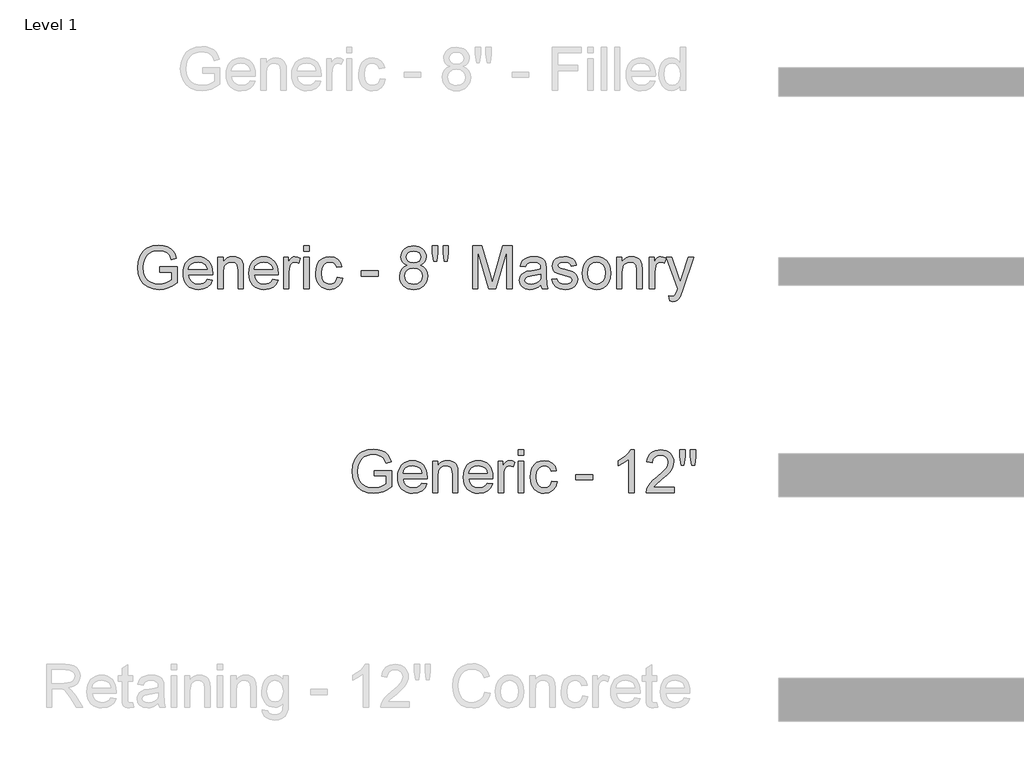
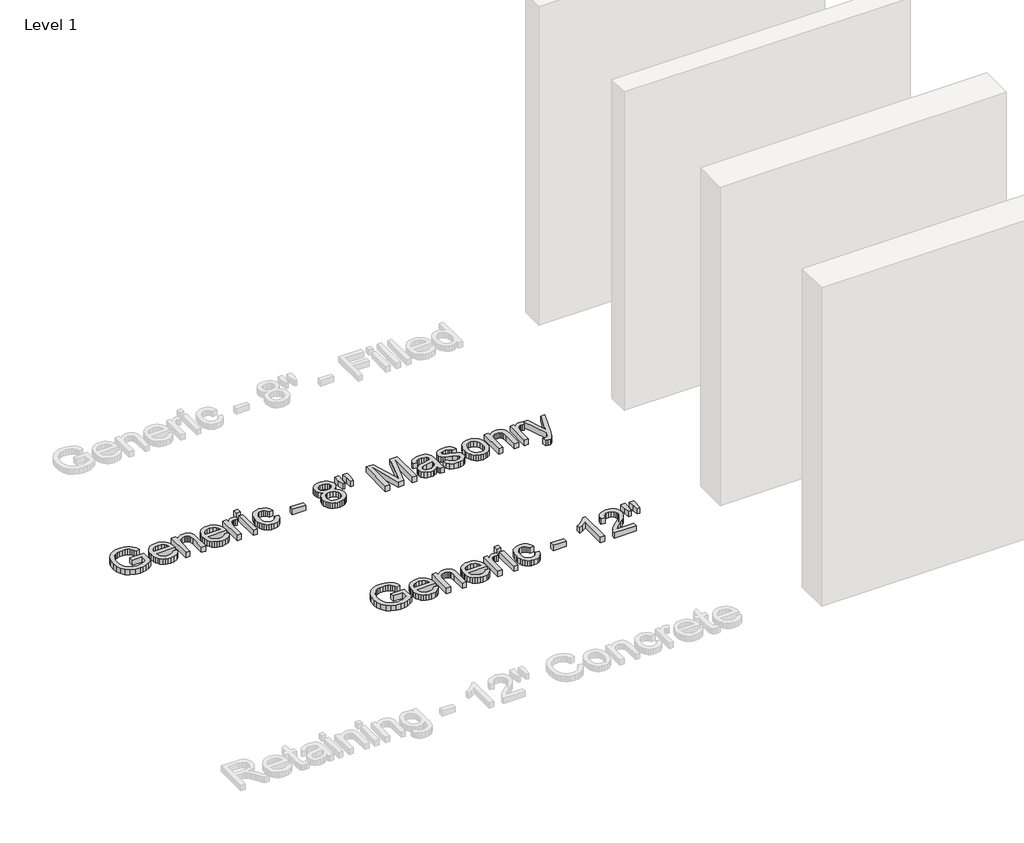
# One storey, part 22 of 42: 2 proxies.
"""IFC4 building model written with IfcOpenShell, lengths in millimetres."""

from ifc_helpers import new_model, si_unit, origin, origin_with_axes, place, context, project, spatial, polyline, outline, extrude, element, save

model = new_model("IFC4")

# Units and contexts
model_context = context("Model", 3, world=origin())
ifc_project = project(units=[si_unit("LENGTHUNIT", "METRE", prefix="MILLI")], contexts=[model_context])

# Site, building, storey
site = spatial("IfcSite", under=ifc_project)
building = spatial("IfcBuilding", under=site)
storey = spatial("IfcBuildingStorey", under=building, Name="Level 1", Elevation=0.0)

# Proxies
placement = place(None, origin())
element("IfcBuildingElementProxy", 1, Name="8\" Arial", ObjectType="8\" Arial", at=placement, inside=storey, context=model_context, shape_type="SweptSolid", body=[
    extrude(outline(polyline([(-16920.0716605, 9639.2549176), (-16920.0716605, 9677.3258044), (-16796.3412786, 9677.3258044), (-16796.3412786, 9563.4849301), (-16826.4094716, 9542.5719674), (-16857.4257189, 9527.5704021), (-16889.3156634, 9518.5360023), (-16922.0049477, 9515.5245356), (-16964.7138649, 9520.3112804), (-17003.3145467, 9534.6715148), (-17035.3810895, 9558.1033277), (-17058.4875896, 9590.1048079), (-17072.4574487, 9628.4917128), (-17077.1140684, 9671.0797995), (-17072.476038, 9713.9746097), (-17058.5619468, 9753.8765425), (-17035.9480632, 9787.3465774), (-17021.5947998, 9800.3800005), (-17005.2106553, 9810.945694), (-16967.7718048, 9824.943437), (-16925.053593, 9829.6093514), (-16893.6934436, 9826.9046082), (-16865.4934752, 9818.7903787), (-16841.7456442, 9805.8522258), (-16823.741907, 9788.6757124), (-16810.4226734, 9766.4336147), (-16800.7283534, 9738.2987089), (-16835.8249521, 9728.4092012), (-16843.6603421, 9748.4763508), (-16853.1873585, 9763.6173358), (-16865.790904, 9775.0311661), (-16882.8558816, 9783.9168516), (-16903.2018706, 9789.6330614), (-16925.6484506, 9791.5384646), (-16951.9244264, 9789.484347), (-16974.3895956, 9783.321994), (-16992.9603065, 9773.8228616), (-17007.5529071, 9761.7584058), (-17027.1460295, 9732.4244901), (-17036.0688936, 9703.685432), (-17039.0431816, 9672.6413007), (-17035.4647414, 9636.2341563), (-17024.7294205, 9606.2774991), (-17007.1625318, 9582.985106), (-16983.0893881, 9566.5707539), (-16954.9173037, 9556.8392553), (-16925.053593, 9553.5954224), (-16898.6846707, 9556.0399154), (-16872.9663739, 9563.3733943), (-16850.6313297, 9573.4766789), (-16834.4121653, 9584.2305891), (-16834.4121653, 9639.2549176), (-16920.0716605, 9639.2549176)])), origin_with_axes(), (0.0, 0.0, 1.0), 50.8),
    extrude(outline(polyline([(-16582.6386837, 9586.9074483), (-16545.311369, 9582.1485875), (-16558.7607277, 9554.0229763), (-16580.2220747, 9532.9984778), (-16609.2120883, 9519.8930212), (-16645.2474467, 9515.5245356), (-16668.8697999, 9517.4090259), (-16689.917535, 9523.0624969), (-16708.3906521, 9532.4849484), (-16724.2891511, 9545.6763805), (-16737.0739423, 9562.2696546), (-16746.205936, 9581.8976319), (-16751.6851322, 9604.5603125), (-16753.5115309, 9630.2576963), (-16751.6665429, 9656.8264536), (-16746.1315788, 9680.2443245), (-16736.9066386, 9700.511309), (-16723.9917223, 9717.6274071), (-16708.1350492, 9731.2254802), (-16690.0848387, 9740.9383896), (-16669.8410909, 9746.7661352), (-16647.4038055, 9748.708717), (-16625.6891793, 9746.7707825), (-16606.0519073, 9740.9569789), (-16588.4919896, 9731.2673061), (-16573.0094262, 9717.7017643), (-16560.3710258, 9700.6228448), (-16551.3435969, 9680.3930389), (-16545.9271396, 9657.0123466), (-16544.1216538, 9630.4807679), (-16544.3447254, 9620.2194742), (-16715.4406442, 9620.2194742), (-16708.8507373, 9591.722077), (-16693.5424486, 9570.7719358), (-16671.4490653, 9557.8895507), (-16644.5038747, 9553.5954224), (-16624.2415375, 9555.5844775), (-16607.17656, 9561.5516429), (-16593.308942, 9571.8687045), (-16582.6386837, 9586.9074483)]), holes=[polyline([(-16715.4406442, 9658.290361), (-16582.1925405, 9658.290361), (-16587.3417767, 9678.4039838), (-16597.4357667, 9692.7921021), (-16619.6313911, 9706.1763982), (-16647.5525199, 9710.6378303), (-16673.2150488, 9707.0779793), (-16694.434735, 9696.3984263), (-16709.1853447, 9679.751708), (-16715.4406442, 9658.290361)])]), origin_with_axes(), (0.0, 0.0, 1.0), 50.8),
    extrude(outline(polyline([(-16506.050767, 9520.2833965), (-16506.050767, 9743.9498562), (-16467.9798803, 9743.9498562), (-16467.9798803, 9712.7198319), (-16454.7535932, 9728.4649691), (-16438.8690362, 9739.7114957), (-16420.3262093, 9746.4594117), (-16399.1251124, 9748.708717), (-16380.3592139, 9746.8962603), (-16363.1734059, 9741.45889), (-16348.8410554, 9733.0751156), (-16338.6355296, 9722.4234466), (-16327.2216993, 9694.4279605), (-16325.2140549, 9657.6211462), (-16325.2140549, 9520.2833965), (-16363.2849417, 9520.2833965), (-16363.2849417, 9652.4904993), (-16367.6720165, 9686.1743112), (-16373.741423, 9696.2032387), (-16383.1754929, 9703.9828608), (-16395.2678326, 9708.9740879), (-16409.3120489, 9710.6378303), (-16431.6099145, 9706.9013809), (-16450.6174739, 9695.6920329), (-16458.2135267, 9686.5414499), (-16463.6392787, 9674.0354982), (-16467.9798803, 9638.9574888), (-16467.9798803, 9520.2833965), (-16506.050767, 9520.2833965)])), origin_with_axes(), (0.0, 0.0, 1.0), 50.8),
    extrude(outline(polyline([(-16116.2703209, 9586.9074483), (-16078.9430062, 9582.1485875), (-16092.3923649, 9554.0229763), (-16113.8537119, 9532.9984778), (-16142.8437255, 9519.8930212), (-16178.8790839, 9515.5245356), (-16202.5014371, 9517.4090259), (-16223.5491723, 9523.0624969), (-16242.0222893, 9532.4849484), (-16257.9207883, 9545.6763805), (-16270.7055795, 9562.2696546), (-16279.8375732, 9581.8976319), (-16285.3167694, 9604.5603125), (-16287.1431682, 9630.2576963), (-16285.2981801, 9656.8264536), (-16279.763216, 9680.2443245), (-16270.5382758, 9700.511309), (-16257.6233595, 9717.6274071), (-16241.7666864, 9731.2254802), (-16223.716476, 9740.9383896), (-16203.4727281, 9746.7661352), (-16181.0354428, 9748.708717), (-16159.3208165, 9746.7707825), (-16139.6835445, 9740.9569789), (-16122.1236268, 9731.2673061), (-16106.6410635, 9717.7017643), (-16094.002663, 9700.6228448), (-16084.9752341, 9680.3930389), (-16079.5587768, 9657.0123466), (-16077.753291, 9630.4807679), (-16077.9763626, 9620.2194742), (-16249.0722814, 9620.2194742), (-16242.4823745, 9591.722077), (-16227.1740858, 9570.7719358), (-16205.0807025, 9557.8895507), (-16178.1355119, 9553.5954224), (-16157.8731747, 9555.5844775), (-16140.8081972, 9561.5516429), (-16126.9405792, 9571.8687045), (-16116.2703209, 9586.9074483)]), holes=[polyline([(-16249.0722814, 9658.290361), (-16115.8241777, 9658.290361), (-16120.9734139, 9678.4039838), (-16131.0674039, 9692.7921021), (-16153.2630283, 9706.1763982), (-16181.1841572, 9710.6378303), (-16206.846686, 9707.0779793), (-16228.0663722, 9696.3984263), (-16242.8169819, 9679.751708), (-16249.0722814, 9658.290361)])]), origin_with_axes(), (0.0, 0.0, 1.0), 50.8),
    extrude(outline(polyline([(-16039.6824042, 9520.2833965), (-16039.6824042, 9743.9498562), (-16006.3703783, 9743.9498562), (-16006.3703783, 9710.8609019), (-15994.0642616, 9730.0450597), (-15982.7247885, 9741.3473542), (-15971.3481368, 9746.8683763), (-15958.9304843, 9748.708717), (-15939.9693981, 9745.7716076), (-15920.7108831, 9736.9602793), (-15933.4259644, 9702.8303242), (-15946.8102605, 9708.6859538), (-15960.1945567, 9710.6378303), (-15971.5619137, 9708.760311), (-15981.7209663, 9703.127753), (-15989.9281423, 9694.1677103), (-15995.4398698, 9682.3077368), (-16000.0686056, 9661.0415774), (-16001.6115175, 9637.8421308), (-16001.6115175, 9520.2833965), (-16039.6824042, 9520.2833965)])), origin_with_axes(), (0.0, 0.0, 1.0), 50.8),
    extrude(outline(polyline([(-15896.9165789, 9786.7796038), (-15896.9165789, 9824.8504905), (-15858.8456921, 9824.8504905), (-15858.8456921, 9786.7796038), (-15896.9165789, 9786.7796038)])), origin_with_axes(), (0.0, 0.0, 1.0), 50.8),
    extrude(outline(polyline([(-15896.9165789, 9520.2833965), (-15896.9165789, 9743.9498562), (-15858.8456921, 9743.9498562), (-15858.8456921, 9520.2833965), (-15896.9165789, 9520.2833965)])), origin_with_axes(), (0.0, 0.0, 1.0), 50.8),
    extrude(outline(polyline([(-15658.9735366, 9601.1840308), (-15620.9026499, 9596.42517), (-15631.5171403, 9562.5647597), (-15651.4634594, 9536.976588), (-15678.8640878, 9520.8875487), (-15711.8415063, 9515.5245356), (-15733.1936413, 9517.395084), (-15752.3382968, 9523.006729), (-15769.2754729, 9532.3594706), (-15784.0051696, 9545.4533089), (-15795.927882, 9562.0419357), (-15804.4441052, 9581.8790426), (-15809.553839, 9604.9646298), (-15811.2570837, 9631.2986971), (-15808.3478582, 9665.1776967), (-15799.6201818, 9694.5394963), (-15784.9346346, 9718.2501487), (-15764.151797, 9735.1757065), (-15739.288608, 9745.3254644), (-15712.3620067, 9748.708717), (-15680.1932228, 9744.061392), (-15654.474926, 9730.1194169), (-15636.0250456, 9707.6263636), (-15625.6615107, 9677.3258044), (-15663.7323975, 9672.5669435), (-15670.6383225, 9689.1764832), (-15681.3922327, 9701.08293), (-15695.3992703, 9708.2491052), (-15712.0645779, 9710.6378303), (-15736.6675167, 9705.9347373), (-15756.1955766, 9691.8254585), (-15768.9385418, 9667.5478325), (-15773.1861969, 9632.3396979), (-15769.0314883, 9596.6575362), (-15756.5673626, 9572.2962584), (-15737.3924994, 9558.2706314), (-15713.1055787, 9553.5954224), (-15693.3916259, 9556.5139425), (-15677.2282294, 9565.2695029), (-15665.4704971, 9580.0851751), (-15658.9735366, 9601.1840308)])), origin_with_axes(), (0.0, 0.0, 1.0), 50.8),
    extrude(outline(polyline([(-15487.6545462, 9610.7017525), (-15487.6545462, 9648.7726393), (-15368.6830251, 9648.7726393), (-15368.6830251, 9610.7017525), (-15487.6545462, 9610.7017525)])), origin_with_axes(), (0.0, 0.0, 1.0), 50.8),
    extrude(outline(polyline([(-15160.9290063, 9688.0332413), (-15181.312174, 9698.0714634), (-15195.6166405, 9711.6788311), (-15204.0654774, 9728.5765049), (-15206.8817564, 9748.4856454), (-15205.3481391, 9764.0123584), (-15200.7472873, 9778.247115), (-15193.079201, 9791.1899153), (-15182.3438802, 9802.8407591), (-15169.0571779, 9812.4700166), (-15153.7349472, 9819.3480577), (-15116.9839007, 9824.8504905), (-15080.0097827, 9819.2179326), (-15064.5202483, 9812.1772352), (-15051.0290637, 9802.3202587), (-15040.0985552, 9790.4416959), (-15032.2910491, 9777.3362393), (-15027.6065455, 9763.0038889), (-15026.0450443, 9747.4446446), (-15028.8241447, 9728.176835), (-15037.1614458, 9711.5672953), (-15051.1498942, 9698.0435794), (-15070.8824363, 9688.0332413), (-15047.4506234, 9675.9594908), (-15030.3949405, 9658.1788252), (-15019.9942271, 9635.5463522), (-15016.5273226, 9608.9171797), (-15018.2468329, 9589.9282096), (-15023.4053637, 9572.51933), (-15032.002915, 9556.6905409), (-15044.0394868, 9542.4418423), (-15058.883043, 9530.6655206), (-15075.9015473, 9522.2538623), (-15095.0949998, 9517.2068673), (-15116.4634003, 9515.5245356), (-15137.8318009, 9517.2138383), (-15157.0252533, 9522.2817462), (-15174.0437576, 9530.7282595), (-15188.8873138, 9542.5533781), (-15200.9238857, 9556.9019942), (-15209.521437, 9572.9189999), (-15214.6799678, 9590.6043954), (-15216.3994781, 9609.9581805), (-15212.7931538, 9637.6190592), (-15201.9741811, 9660.3723626), (-15184.500239, 9677.4373402), (-15160.9290063, 9688.0332413)]), holes=[polyline([(-15168.8108696, 9747.3702874), (-15165.4369116, 9730.7514531), (-15155.3150377, 9717.4786927), (-15138.7426766, 9708.7789003), (-15116.0172571, 9705.8789694), (-15093.8216327, 9708.760311), (-15077.5002272, 9717.4043355), (-15067.4620051, 9730.2309527), (-15064.115931, 9745.6600718), (-15067.5735409, 9761.6747539), (-15077.9463704, 9774.9196303), (-15094.4908475, 9783.8146104), (-15116.4634003, 9786.7796038), (-15138.5753729, 9783.879673), (-15155.0919661, 9775.1798805), (-15165.3811437, 9762.4276206), (-15168.8108696, 9747.3702874)]), polyline([(-15178.3285913, 9611.2966101), (-15176.7392061, 9596.7318934), (-15171.9710507, 9582.6319093), (-15163.169017, 9570.3350872), (-15149.4779974, 9561.1798569), (-15133.0822347, 9555.491531), (-15116.1659715, 9553.5954224), (-15090.2524871, 9557.5828273), (-15070.8080791, 9569.5450419), (-15058.6506768, 9587.660315), (-15054.5982093, 9610.1068949), (-15058.7808019, 9632.9345555), (-15071.3285795, 9651.4494985), (-15091.2191307, 9663.7184366), (-15117.4300439, 9667.8080827), (-15142.981037, 9663.7742045), (-15162.2302574, 9651.6725701), (-15174.3040078, 9633.5108238), (-15178.3285913, 9611.2966101)])]), origin_with_axes(), (0.0, 0.0, 1.0), 50.8),
    extrude(outline(polyline([(-14973.9206466, 9715.3966911), (-14983.2152967, 9774.2132369), (-14983.2152967, 9824.8504905), (-14945.1444099, 9824.8504905), (-14945.1444099, 9774.2132369), (-14953.4724164, 9715.3966911), (-14973.9206466, 9715.3966911)])), origin_with_axes(), (0.0, 0.0, 1.0), 50.8),
    extrude(outline(polyline([(-14898.0019447, 9715.3966911), (-14907.0735232, 9774.2132369), (-14907.0735232, 9824.8504905), (-14869.0026364, 9824.8504905), (-14869.0026364, 9774.2132369), (-14877.9255005, 9715.3966911), (-14898.0019447, 9715.3966911)])), origin_with_axes(), (0.0, 0.0, 1.0), 50.8),
    extrude(outline(polyline([(-14697.683646, 9520.2833965), (-14697.683646, 9824.8504905), (-14632.1749522, 9824.8504905), (-14569.863618, 9610.1812521), (-14557.2972511, 9565.3438601), (-14543.6898833, 9613.8991122), (-14482.41955, 9824.8504905), (-14416.9108561, 9824.8504905), (-14416.9108561, 9520.2833965), (-14454.9817429, 9520.2833965), (-14454.9817429, 9786.7796038), (-14531.4953024, 9520.2833965), (-14583.0991997, 9520.2833965), (-14659.6127592, 9786.7796038), (-14659.6127592, 9520.2833965), (-14697.683646, 9520.2833965)])), origin_with_axes(), (0.0, 0.0, 1.0), 50.8),
    extrude(outline(polyline([(-14212.2798398, 9548.8365615), (-14230.46947, 9533.2401387), (-14249.19819, 9523.0346129), (-14268.8935535, 9517.402055), (-14289.9831145, 9515.5245356), (-14321.7987018, 9520.0417356), (-14345.2676933, 9533.5933354), (-14359.7394635, 9554.1716907), (-14364.5633868, 9579.769157), (-14362.7416354, 9595.5514729), (-14357.2763812, 9609.8838233), (-14348.8461336, 9622.1527614), (-14338.129402, 9631.7448403), (-14311.4723455, 9644.23685), (-14278.5321056, 9649.9623545), (-14239.6061111, 9655.9852878), (-14212.5029114, 9663.0492218), (-14212.2798398, 9671.5259427), (-14214.9009311, 9688.5165631), (-14222.7642051, 9699.6329646), (-14240.3496831, 9707.8866138), (-14264.8503807, 9710.6378303), (-14287.5293269, 9708.8067842), (-14303.3674107, 9703.313646), (-14314.1677941, 9693.1545935), (-14321.7336392, 9677.3258044), (-14359.804526, 9682.0846652), (-14353.1960298, 9702.9046814), (-14343.334406, 9719.2632656), (-14329.2994844, 9731.7738646), (-14310.1710945, 9741.0499254), (-14286.7764603, 9746.7940191), (-14259.9428055, 9748.708717), (-14234.2059194, 9747.0170907), (-14213.8041624, 9741.9422118), (-14198.4215165, 9734.311304), (-14187.7419636, 9724.9515914), (-14180.6594402, 9713.379752), (-14176.0678831, 9699.1124642), (-14174.2089531, 9665.8004382), (-14174.2089531, 9618.4349014), (-14172.2756658, 9552.2941714), (-14164.6912314, 9520.2833965), (-14202.7621181, 9520.2833965), (-14208.8594086, 9533.5189782), (-14212.2798398, 9548.8365615)]), holes=[polyline([(-14212.2798398, 9624.9783351), (-14273.6988876, 9613.3042546), (-14306.4532345, 9607.1326069), (-14321.287496, 9597.0943848), (-14326.4925001, 9582.4460163), (-14323.6576318, 9571.1251325), (-14315.153027, 9561.8490717), (-14301.1645786, 9555.6588347), (-14281.8781797, 9553.5954224), (-14261.4299495, 9555.8726117), (-14243.3611497, 9562.7041795), (-14228.7127812, 9572.7702855), (-14218.5258447, 9584.7510895), (-14214.0086447, 9597.0943848), (-14212.5029114, 9614.196541), (-14212.2798398, 9624.9783351)])]), origin_with_axes(), (0.0, 0.0, 1.0), 50.8),
    extrude(outline(polyline([(-14136.1380663, 9586.9074483), (-14098.0671795, 9591.6663091), (-14092.0628356, 9575.3820822), (-14080.444523, 9563.4105729), (-14063.1378845, 9556.04921), (-14040.068563, 9553.5954224), (-14017.278081, 9555.8447277), (-14001.2541042, 9562.5926437), (-13991.7735611, 9572.3706156), (-13988.6133801, 9583.7100887), (-13991.7921504, 9593.4137034), (-14001.3284614, 9600.8122448), (-14040.5147062, 9611.6683961), (-14097.8441079, 9630.2948749), (-14112.3530567, 9639.6545876), (-14122.865306, 9652.0443561), (-14129.2507306, 9666.6741354), (-14131.3792055, 9682.75388), (-14129.6689898, 9697.5044897), (-14124.538343, 9711.1211521), (-14116.4519974, 9723.0647774), (-14105.8746856, 9732.7962761), (-14081.6714168, 9744.061392), (-14048.9170699, 9748.708717), (-14024.1375327, 9746.8404924), (-14002.5925338, 9741.2358184), (-13985.2673061, 9732.4430794), (-13973.1470824, 9721.0106598), (-13965.1165047, 9706.0927464), (-13960.060215, 9686.843526), (-13998.1311018, 9682.0846652), (-14002.9364359, 9694.0654692), (-14012.4448629, 9703.0905744), (-14026.7493294, 9708.7510163), (-14045.9427818, 9710.6378303), (-14067.8037989, 9708.8346682), (-14082.3778102, 9703.4251818), (-14090.5756916, 9695.6176757), (-14093.3083187, 9686.6204544), (-14088.7725295, 9675.5412315), (-14074.5703041, 9667.1388679), (-14041.7787786, 9659.033933), (-13985.8993423, 9641.1138476), (-13971.1394379, 9632.5441802), (-13959.9486792, 9620.8143318), (-13952.8940398, 9605.8871238), (-13950.5424933, 9587.7253775), (-13953.3030044, 9568.9501843), (-13961.5845377, 9551.2903492), (-13975.0710749, 9536.1307749), (-13993.4465982, 9524.8563643), (-14015.6422226, 9517.8574928), (-14040.5890634, 9515.5245356), (-14078.9759683, 9520.0231463), (-14106.9900436, 9533.5189782), (-14125.6908796, 9555.863317), (-14136.1380663, 9586.9074483)])), origin_with_axes(), (0.0, 0.0, 1.0), 50.8),
    extrude(outline(polyline([(-13917.2304674, 9632.1166263), (-13915.1717024, 9661.0834033), (-13908.9954075, 9686.0441861), (-13898.7015825, 9706.9989748), (-13884.2902275, 9723.9477692), (-13869.7812787, 9734.7806839), (-13853.7665966, 9742.5184801), (-13836.2461812, 9747.1611578), (-13817.2200325, 9748.708717), (-13796.216447, 9746.8242267), (-13777.2251532, 9741.1707558), (-13760.2461511, 9731.7483043), (-13745.2794408, 9718.5568721), (-13733.0639469, 9702.0426026), (-13724.3385942, 9682.6516389), (-13719.1033825, 9660.3839809), (-13717.358312, 9635.2396288), (-13720.4441358, 9596.7783667), (-13729.7016073, 9567.5002189), (-13744.8611816, 9545.5741394), (-13765.6533138, 9529.169082), (-13790.3491991, 9518.9356722), (-13817.2200325, 9515.5245356), (-13838.5303415, 9517.402055), (-13857.6982336, 9523.0346129), (-13874.7237089, 9532.4222095), (-13889.6067674, 9545.5648447), (-13901.6921362, 9562.239447), (-13910.3245424, 9582.2229447), (-13915.5039862, 9605.5153378), (-13917.2304674, 9632.1166263)]), holes=[polyline([(-13879.1595807, 9632.1909835), (-13874.7539165, 9597.7357157), (-13861.5369241, 9573.1885448), (-13841.6463729, 9558.493703), (-13817.2200325, 9553.5954224), (-13792.9052279, 9558.5215869), (-13773.0518553, 9573.3000806), (-13759.8348629, 9598.1725642), (-13755.4291987, 9633.3806987), (-13759.8627468, 9666.8321444), (-13773.1633911, 9691.0447079), (-13793.0446476, 9705.7395497), (-13817.2200325, 9710.6378303), (-13841.6463729, 9705.758139), (-13861.5369241, 9691.1190651), (-13874.7539165, 9666.6276621), (-13879.1595807, 9632.1909835)])]), origin_with_axes(), (0.0, 0.0, 1.0), 50.8),
    extrude(outline(polyline([(-13674.5285644, 9520.2833965), (-13674.5285644, 9743.9498562), (-13636.4576776, 9743.9498562), (-13636.4576776, 9712.7198319), (-13623.2313905, 9728.4649691), (-13607.3468335, 9739.7114957), (-13588.8040066, 9746.4594117), (-13567.6029097, 9748.708717), (-13548.8370112, 9746.8962603), (-13531.6512032, 9741.45889), (-13517.3188528, 9733.0751156), (-13507.113327, 9722.4234466), (-13495.6994967, 9694.4279605), (-13493.6918522, 9657.6211462), (-13493.6918522, 9520.2833965), (-13531.762739, 9520.2833965), (-13531.762739, 9652.4904993), (-13536.1498138, 9686.1743112), (-13542.2192204, 9696.2032387), (-13551.6532902, 9703.9828608), (-13563.74563, 9708.9740879), (-13577.7898462, 9710.6378303), (-13600.0877118, 9706.9013809), (-13619.0952712, 9695.6920329), (-13626.691324, 9686.5414499), (-13632.117076, 9674.0354982), (-13636.4576776, 9638.9574888), (-13636.4576776, 9520.2833965), (-13674.5285644, 9520.2833965)])), origin_with_axes(), (0.0, 0.0, 1.0), 50.8),
    extrude(outline(polyline([(-13441.344383, 9520.2833965), (-13441.344383, 9743.9498562), (-13408.032357, 9743.9498562), (-13408.032357, 9710.8609019), (-13395.7262403, 9730.0450597), (-13384.3867672, 9741.3473542), (-13373.0101155, 9746.8683763), (-13360.592463, 9748.708717), (-13341.6313768, 9745.7716076), (-13322.3728618, 9736.9602793), (-13335.0879432, 9702.8303242), (-13348.4722393, 9708.6859538), (-13361.8565354, 9710.6378303), (-13373.2238925, 9708.760311), (-13383.382945, 9703.127753), (-13391.590121, 9694.1677103), (-13397.1018485, 9682.3077368), (-13401.7305843, 9661.0415774), (-13403.2734962, 9637.8421308), (-13403.2734962, 9520.2833965), (-13441.344383, 9520.2833965)])), origin_with_axes(), (0.0, 0.0, 1.0), 50.8),
    extrude(outline(polyline([(-13298.5785576, 9434.6239013), (-13303.3374185, 9471.2820012), (-13284.0045463, 9467.9359272), (-13265.9357465, 9472.137109), (-13254.8565236, 9483.8483681), (-13244.4465155, 9511.8810328), (-13241.4722275, 9521.1013257), (-13322.3728618, 9743.9498562), (-13282.2199735, 9743.9498562), (-13239.3158687, 9619.773331), (-13224.3700713, 9570.1027209), (-13209.424274, 9613.9734694), (-13165.330454, 9743.9498562), (-13125.4749944, 9743.9498562), (-13203.3269835, 9514.929678), (-13223.5521421, 9465.259068), (-13233.9063823, 9449.4023949), (-13245.6362307, 9438.4161185), (-13259.2621877, 9432.0028099), (-13275.3047538, 9429.8650404), (-13298.5785576, 9434.6239013)])), origin_with_axes(), (0.0, 0.0, 1.0), 50.8),
])
element("IfcBuildingElementProxy", 2, Name="8\" Arial", ObjectType="8\" Arial", at=placement, inside=storey, context=model_context, shape_type="SweptSolid", body=[
    extrude(outline(polyline([(-15396.0716605, 8191.4549176), (-15396.0716605, 8229.5258044), (-15272.3412786, 8229.5258044), (-15272.3412786, 8115.6849301), (-15302.4094716, 8094.7719674), (-15333.4257189, 8079.7704021), (-15365.3156634, 8070.7360023), (-15398.0049477, 8067.7245356), (-15440.7138649, 8072.5112804), (-15479.3145467, 8086.8715148), (-15511.3810895, 8110.3033277), (-15534.4875896, 8142.3048079), (-15548.4574487, 8180.6917128), (-15553.1140684, 8223.2797995), (-15548.476038, 8266.1746097), (-15534.5619468, 8306.0765425), (-15511.9480632, 8339.5465774), (-15497.5947998, 8352.5800005), (-15481.2106553, 8363.145694), (-15443.7718048, 8377.143437), (-15401.053593, 8381.8093514), (-15369.6934436, 8379.1046082), (-15341.4934752, 8370.9903787), (-15317.7456442, 8358.0522258), (-15299.741907, 8340.8757124), (-15286.4226734, 8318.6336147), (-15276.7283534, 8290.4987089), (-15311.8249521, 8280.6092012), (-15319.6603421, 8300.6763508), (-15329.1873585, 8315.8173358), (-15341.790904, 8327.2311661), (-15358.8558816, 8336.1168516), (-15379.2018706, 8341.8330614), (-15401.6484506, 8343.7384646), (-15427.9244264, 8341.684347), (-15450.3895956, 8335.521994), (-15468.9603065, 8326.0228616), (-15483.5529071, 8313.9584058), (-15503.1460295, 8284.6244901), (-15512.0688936, 8255.885432), (-15515.0431816, 8224.8413007), (-15511.4647414, 8188.4341563), (-15500.7294205, 8158.4774991), (-15483.1625318, 8135.185106), (-15459.0893881, 8118.7707539), (-15430.9173037, 8109.0392553), (-15401.053593, 8105.7954224), (-15374.6846707, 8108.2399154), (-15348.9663739, 8115.5733943), (-15326.6313297, 8125.6766789), (-15310.4121653, 8136.4305891), (-15310.4121653, 8191.4549176), (-15396.0716605, 8191.4549176)])), origin_with_axes(), (0.0, 0.0, 1.0), 50.8),
    extrude(outline(polyline([(-15058.6386837, 8139.1074483), (-15021.311369, 8134.3485875), (-15034.7607277, 8106.2229763), (-15056.2220747, 8085.1984778), (-15085.2120883, 8072.0930212), (-15121.2474467, 8067.7245356), (-15144.8697999, 8069.6090259), (-15165.917535, 8075.2624969), (-15184.3906521, 8084.6849484), (-15200.2891511, 8097.8763805), (-15213.0739423, 8114.4696546), (-15222.205936, 8134.0976319), (-15227.6851322, 8156.7603125), (-15229.5115309, 8182.4576963), (-15227.6665429, 8209.0264536), (-15222.1315788, 8232.4443245), (-15212.9066386, 8252.711309), (-15199.9917223, 8269.8274071), (-15184.1350492, 8283.4254802), (-15166.0848387, 8293.1383896), (-15145.8410909, 8298.9661352), (-15123.4038055, 8300.908717), (-15101.6891793, 8298.9707825), (-15082.0519073, 8293.1569789), (-15064.4919896, 8283.4673061), (-15049.0094262, 8269.9017643), (-15036.3710258, 8252.8228448), (-15027.3435969, 8232.5930389), (-15021.9271396, 8209.2123466), (-15020.1216538, 8182.6807679), (-15020.3447254, 8172.4194742), (-15191.4406442, 8172.4194742), (-15184.8507373, 8143.922077), (-15169.5424486, 8122.9719358), (-15147.4490653, 8110.0895507), (-15120.5038747, 8105.7954224), (-15100.2415375, 8107.7844775), (-15083.17656, 8113.7516429), (-15069.308942, 8124.0687045), (-15058.6386837, 8139.1074483)]), holes=[polyline([(-15191.4406442, 8210.490361), (-15058.1925405, 8210.490361), (-15063.3417767, 8230.6039838), (-15073.4357667, 8244.9921021), (-15095.6313911, 8258.3763982), (-15123.5525199, 8262.8378303), (-15149.2150488, 8259.2779793), (-15170.434735, 8248.5984263), (-15185.1853447, 8231.951708), (-15191.4406442, 8210.490361)])]), origin_with_axes(), (0.0, 0.0, 1.0), 50.8),
    extrude(outline(polyline([(-14982.050767, 8072.4833965), (-14982.050767, 8296.1498562), (-14943.9798803, 8296.1498562), (-14943.9798803, 8264.9198319), (-14930.7535932, 8280.6649691), (-14914.8690362, 8291.9114957), (-14896.3262093, 8298.6594117), (-14875.1251124, 8300.908717), (-14856.3592139, 8299.0962603), (-14839.1734059, 8293.65889), (-14824.8410554, 8285.2751156), (-14814.6355296, 8274.6234466), (-14803.2216993, 8246.6279605), (-14801.2140549, 8209.8211462), (-14801.2140549, 8072.4833965), (-14839.2849417, 8072.4833965), (-14839.2849417, 8204.6904993), (-14843.6720165, 8238.3743112), (-14849.741423, 8248.4032387), (-14859.1754929, 8256.1828608), (-14871.2678326, 8261.1740879), (-14885.3120489, 8262.8378303), (-14907.6099145, 8259.1013809), (-14926.6174739, 8247.8920329), (-14934.2135267, 8238.7414499), (-14939.6392787, 8226.2354982), (-14943.9798803, 8191.1574888), (-14943.9798803, 8072.4833965), (-14982.050767, 8072.4833965)])), origin_with_axes(), (0.0, 0.0, 1.0), 50.8),
    extrude(outline(polyline([(-14592.2703209, 8139.1074483), (-14554.9430062, 8134.3485875), (-14568.3923649, 8106.2229763), (-14589.8537119, 8085.1984778), (-14618.8437255, 8072.0930212), (-14654.8790839, 8067.7245356), (-14678.5014371, 8069.6090259), (-14699.5491723, 8075.2624969), (-14718.0222893, 8084.6849484), (-14733.9207883, 8097.8763805), (-14746.7055795, 8114.4696546), (-14755.8375732, 8134.0976319), (-14761.3167694, 8156.7603125), (-14763.1431682, 8182.4576963), (-14761.2981801, 8209.0264536), (-14755.763216, 8232.4443245), (-14746.5382758, 8252.711309), (-14733.6233595, 8269.8274071), (-14717.7666864, 8283.4254802), (-14699.716476, 8293.1383896), (-14679.4727281, 8298.9661352), (-14657.0354428, 8300.908717), (-14635.3208165, 8298.9707825), (-14615.6835445, 8293.1569789), (-14598.1236268, 8283.4673061), (-14582.6410635, 8269.9017643), (-14570.002663, 8252.8228448), (-14560.9752341, 8232.5930389), (-14555.5587768, 8209.2123466), (-14553.753291, 8182.6807679), (-14553.9763626, 8172.4194742), (-14725.0722814, 8172.4194742), (-14718.4823745, 8143.922077), (-14703.1740858, 8122.9719358), (-14681.0807025, 8110.0895507), (-14654.1355119, 8105.7954224), (-14633.8731747, 8107.7844775), (-14616.8081972, 8113.7516429), (-14602.9405792, 8124.0687045), (-14592.2703209, 8139.1074483)]), holes=[polyline([(-14725.0722814, 8210.490361), (-14591.8241777, 8210.490361), (-14596.9734139, 8230.6039838), (-14607.0674039, 8244.9921021), (-14629.2630283, 8258.3763982), (-14657.1841572, 8262.8378303), (-14682.846686, 8259.2779793), (-14704.0663722, 8248.5984263), (-14718.8169819, 8231.951708), (-14725.0722814, 8210.490361)])]), origin_with_axes(), (0.0, 0.0, 1.0), 50.8),
    extrude(outline(polyline([(-14515.6824042, 8072.4833965), (-14515.6824042, 8296.1498562), (-14482.3703783, 8296.1498562), (-14482.3703783, 8263.0609019), (-14470.0642616, 8282.2450597), (-14458.7247885, 8293.5473542), (-14447.3481368, 8299.0683763), (-14434.9304843, 8300.908717), (-14415.9693981, 8297.9716076), (-14396.7108831, 8289.1602793), (-14409.4259644, 8255.0303242), (-14422.8102605, 8260.8859538), (-14436.1945567, 8262.8378303), (-14447.5619137, 8260.960311), (-14457.7209663, 8255.327753), (-14465.9281423, 8246.3677103), (-14471.4398698, 8234.5077368), (-14476.0686056, 8213.2415774), (-14477.6115175, 8190.0421308), (-14477.6115175, 8072.4833965), (-14515.6824042, 8072.4833965)])), origin_with_axes(), (0.0, 0.0, 1.0), 50.8),
    extrude(outline(polyline([(-14372.9165789, 8338.9796038), (-14372.9165789, 8377.0504905), (-14334.8456921, 8377.0504905), (-14334.8456921, 8338.9796038), (-14372.9165789, 8338.9796038)])), origin_with_axes(), (0.0, 0.0, 1.0), 50.8),
    extrude(outline(polyline([(-14372.9165789, 8072.4833965), (-14372.9165789, 8296.1498562), (-14334.8456921, 8296.1498562), (-14334.8456921, 8072.4833965), (-14372.9165789, 8072.4833965)])), origin_with_axes(), (0.0, 0.0, 1.0), 50.8),
    extrude(outline(polyline([(-14134.9735366, 8153.3840308), (-14096.9026499, 8148.62517), (-14107.5171403, 8114.7647597), (-14127.4634594, 8089.176588), (-14154.8640878, 8073.0875487), (-14187.8415063, 8067.7245356), (-14209.1936413, 8069.595084), (-14228.3382968, 8075.206729), (-14245.2754729, 8084.5594706), (-14260.0051696, 8097.6533089), (-14271.927882, 8114.2419357), (-14280.4441052, 8134.0790426), (-14285.553839, 8157.1646298), (-14287.2570837, 8183.4986971), (-14284.3478582, 8217.3776967), (-14275.6201818, 8246.7394963), (-14260.9346346, 8270.4501487), (-14240.151797, 8287.3757065), (-14215.288608, 8297.5254644), (-14188.3620067, 8300.908717), (-14156.1932228, 8296.261392), (-14130.474926, 8282.3194169), (-14112.0250456, 8259.8263636), (-14101.6615107, 8229.5258044), (-14139.7323975, 8224.7669435), (-14146.6383225, 8241.3764832), (-14157.3922327, 8253.28293), (-14171.3992703, 8260.4491052), (-14188.0645779, 8262.8378303), (-14212.6675167, 8258.1347373), (-14232.1955766, 8244.0254585), (-14244.9385418, 8219.7478325), (-14249.1861969, 8184.5396979), (-14245.0314883, 8148.8575362), (-14232.5673626, 8124.4962584), (-14213.3924994, 8110.4706314), (-14189.1055787, 8105.7954224), (-14169.3916259, 8108.7139425), (-14153.2282294, 8117.4695029), (-14141.4704971, 8132.2851751), (-14134.9735366, 8153.3840308)])), origin_with_axes(), (0.0, 0.0, 1.0), 50.8),
    extrude(outline(polyline([(-13963.6545462, 8162.9017525), (-13963.6545462, 8200.9726393), (-13844.6830251, 8200.9726393), (-13844.6830251, 8162.9017525), (-13963.6545462, 8162.9017525)])), origin_with_axes(), (0.0, 0.0, 1.0), 50.8),
    extrude(outline(polyline([(-13549.6336527, 8072.4833965), (-13587.7045395, 8072.4833965), (-13587.7045395, 8309.8315811), (-13623.7677818, 8284.1411683), (-13663.846313, 8264.9198319), (-13663.846313, 8300.908717), (-13633.9454237, 8317.1743547), (-13608.0412339, 8336.5258162), (-13587.6208876, 8357.1041715), (-13574.171529, 8377.0504905), (-13549.6336527, 8377.0504905), (-13549.6336527, 8072.4833965)])), origin_with_axes(), (0.0, 0.0, 1.0), 50.8),
    extrude(outline(polyline([(-13264.102002, 8110.5542832), (-13264.102002, 8072.4833965), (-13463.9741575, 8072.4833965), (-13459.8845115, 8098.7314883), (-13450.4969149, 8119.2447811), (-13436.7594221, 8139.1446269), (-13416.8874602, 8159.9739378), (-13389.0964564, 8183.2756255), (-13348.014103, 8219.7664218), (-13323.364691, 8246.7023177), (-13311.039985, 8268.5633347), (-13306.9317496, 8289.8294941), (-13310.8076187, 8308.8928215), (-13322.435226, 8324.7401999), (-13340.3088381, 8335.4197528), (-13362.9227218, 8338.9796038), (-13386.6705527, 8335.5034047), (-13405.1204332, 8325.0748073), (-13417.0268799, 8308.5117408), (-13421.1444099, 8286.6321345), (-13459.2152967, 8291.3909953), (-13455.9412562, 8311.0445329), (-13449.9857091, 8328.216399), (-13441.3486555, 8342.9065934), (-13430.0300954, 8355.1151163), (-13416.2902789, 8364.7118426), (-13400.3894563, 8371.566647), (-13362.1047926, 8377.0504905), (-13341.700712, 8375.5261679), (-13323.5412893, 8370.9532001), (-13307.6265247, 8363.331587), (-13293.9564181, 8352.6613287), (-13282.9771127, 8339.7324704), (-13275.1347517, 8325.3350575), (-13270.4293351, 8309.4690898), (-13268.8608629, 8292.1345673), (-13270.5524892, 8273.9263478), (-13275.6273681, 8256.0341464), (-13284.6338841, 8237.8352215), (-13298.1204214, 8218.7068317), (-13319.618947, 8195.8698764), (-13352.6614281, 8166.5452554), (-13396.4578193, 8129.924334), (-13413.6343326, 8110.5542832), (-13264.102002, 8110.5542832)])), origin_with_axes(), (0.0, 0.0, 1.0), 50.8),
    extrude(outline(polyline([(-13216.7364652, 8267.5966911), (-13226.0311153, 8326.4132369), (-13226.0311153, 8377.0504905), (-13187.9602285, 8377.0504905), (-13187.9602285, 8326.4132369), (-13196.288235, 8267.5966911), (-13216.7364652, 8267.5966911)])), origin_with_axes(), (0.0, 0.0, 1.0), 50.8),
    extrude(outline(polyline([(-13140.8177633, 8267.5966911), (-13149.8893418, 8326.4132369), (-13149.8893418, 8377.0504905), (-13111.818455, 8377.0504905), (-13111.818455, 8326.4132369), (-13120.7413191, 8267.5966911), (-13140.8177633, 8267.5966911)])), origin_with_axes(), (0.0, 0.0, 1.0), 50.8),
])

save(model, "model.ifc")

# Revit data of these elements
# Elements 1, 2 (IfcBuildingElementProxy, "8\" Arial")
#   Phase Created = New Construction
